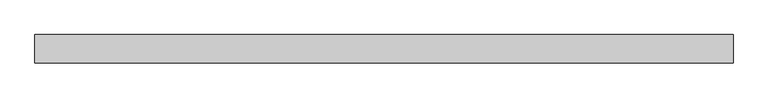
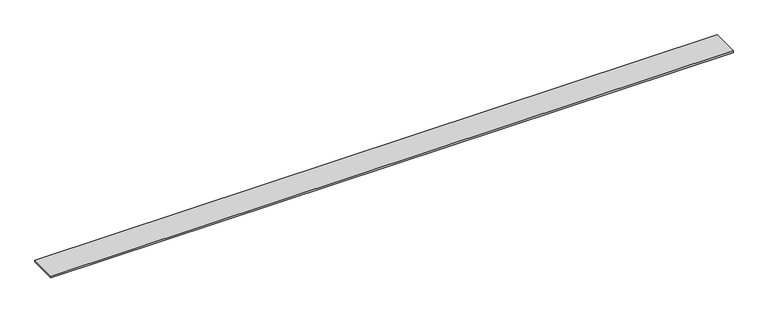
"""IFC4 building model written with IfcOpenShell, lengths in millimetres: proxy geometry, Generic Models 7:Generic Models 1:5:Generic Models 1:5 : Generic Models 7:Generic Models 1:337419:5 : Generic Models 7:Generic Models 1:5:Generic Models 1:5 : Generic Models 7:Generic Models 1:337419:311462."""

from ifc_helpers import new_model, si_unit, frame, origin, place, context, project, spatial, polyline, outline, extrude, source, transform, mapped, element, save


def generic_models_298e8039(model_context):
    return source(origin(), model_context, "Body", "SweptSolid", [
        extrude(outline(polyline([(570452.6367239, -579004.6336751), (570452.6367239, -579104.1113296), (568007.8867239, -579104.1113296), (568007.8867239, -579004.6336751), (570452.6367239, -579004.6336751)])), frame((0.0, 0.0, 3704.43125), z_axis=(0.0, 0.0, 1.0), x_axis=(1.0, 0.0, 0.0)), (0.0, 0.0, 1.0), 6.35),
    ])


if __name__ == "__main__":
    model = new_model("IFC4")
    model_context = context("Model", 3, world=origin())
    ifc_project = project(units=[si_unit("LENGTHUNIT", "METRE", prefix="MILLI")], contexts=[model_context])
    site = spatial("IfcSite", under=ifc_project)
    building = spatial("IfcBuilding", under=site)
    placement = place(None, origin())
    generic_models_shape = generic_models_298e8039(model_context)
    element("IfcBuildingElementProxy", 1, Name="Generic Models 7:Generic Models 1:5:Generic Models 1:5 : Generic Models 7:Generic Models 1:337419:5 : Generic Models 7:Generic Models 1:5:Generic Models 1:5 : Generic Models 7:Generic Models 1:337419:311462", ObjectType="Generic Models 7:Generic Models 1:5:Generic Models 1:5 : Generic Models 7:Generic Models 1:337419:5 : Generic Models 7:Generic Models 1:5:Generic Models 1:5 : Generic Models 7:Generic Models 1:337419:311462", at=placement, inside=building, context=model_context, shape_type="MappedRepresentation", body=[
        mapped(generic_models_shape, transform((0.0, 0.0, 0.0), x_axis=(1.0, 0.0, 0.0), y_axis=(0.0, 1.0, 0.0), z_axis=(0.0, 0.0, 1.0))),
    ])
    save(model, "model.ifc")

# Revit data of these elements
# Type "Generic Models 7:Generic Models 1:5:Generic Models 1:5 : Generic Models 7:Generic Models 1:337419:5 : Generic Models 7:Generic Models 1:5:Generic Models 1:5 : Generic Models 7:Generic Models 1:337419:311462"
#   NameOverride = "Generic Models 7:Generic Models 1:5:Generic Models 1:5 : Generic Models 7:Generic Models 1:337419:311462"
#   ObjectTypeOverride = "Generic Models 1:5 : Generic Models 7:Generic Models 1:337419"
#   Reference = "Generic Models 1"
#   Tag = "311462"
# Element 1 (IfcBuildingElementProxy, "Generic Models 7:Generic Models 1:5:Generic Models 1:5 : Generic Models 7:Generic Models 1:337419:5 : Generic Models 7:Generic Models 1:5:Generic Models 1:5 : Generic Models 7:Generic Models 1:337419:311462")
#   Materials on its faces: "WOOD BLOCKING - SIZE AS NECESSARY"
# Materials
#   "WOOD BLOCKING - SIZE AS NECESSARY": class "Wood", colour RGB 144 113 62, transparency 0, Description = "Pinus Echinata", Cost = 0
